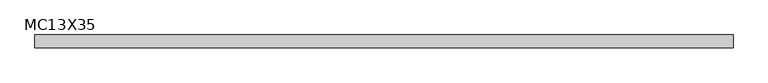
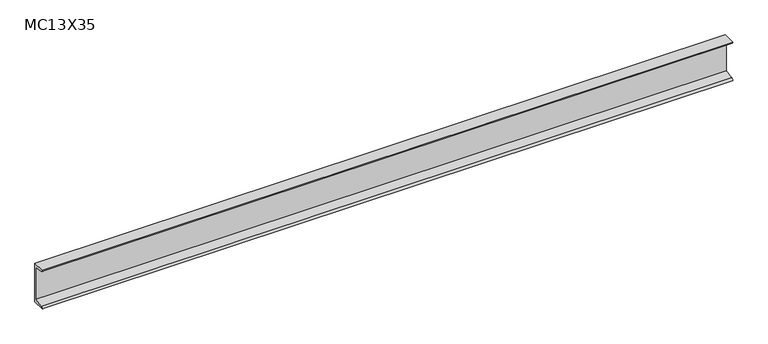
"""IFC4 building model written with IfcOpenShell, lengths in millimetres: beam geometry, MC-Miscellaneous Channel : MC13X35."""

from ifc_helpers import new_model, si_unit, point, frame, frame_2d, origin, place, context, project, spatial, polyline, circle_curve, trimmed, segment, composite_curve, outline, extrude, source, transform, mapped, element, save


def mc13x35_d1883c7b(model_context):
    return source(origin(), model_context, "Body", "SweptSolid", [
        extrude(outline(composite_curve([segment(polyline([(24.892, 165.1), (24.892, -165.1), (-78.486, -165.1)]), True, "CONTINUOUS"), segment(trimmed(circle_curve(frame_2d((-62.992, -165.1)), 15.494), [point((-78.486, -165.1))], [point((-62.992, -149.606))], False, "CARTESIAN"), True, "CONTINUOUS"), segment(polyline([(-62.992, -149.606), (13.5382, -137.4848071), (13.5382, 137.4848071), (-62.992, 149.606)]), True, "CONTINUOUS"), segment(trimmed(circle_curve(frame_2d((-62.992, 165.1)), 15.494), [point((-62.992, 149.606))], [point((-78.486, 165.1))], False, "CARTESIAN"), True, "CONTINUOUS"), segment(polyline([(-78.486, 165.1), (24.892, 165.1)]), True, "CONTINUOUS")], self_intersect=False)), frame((-2806.7, 0.0, 0.0), z_axis=(1.0, 0.0, 0.0), x_axis=(0.0, 1.0, 0.0)), (0.0, 0.0, 1.0), 5613.4),
    ])


if __name__ == "__main__":
    model = new_model("IFC4")
    model_context = context("Model", 3, world=origin())
    ifc_project = project(units=[si_unit("LENGTHUNIT", "METRE", prefix="MILLI")], contexts=[model_context])
    site = spatial("IfcSite", under=ifc_project)
    building = spatial("IfcBuilding", under=site)
    placement = place(None, origin())
    mc13x35_shape = mc13x35_d1883c7b(model_context)
    element("IfcBeam", 1, ObjectType="MC-Miscellaneous Channel : MC13X35", at=placement, inside=building, context=model_context, shape_type="MappedRepresentation", body=[
        mapped(mc13x35_shape, transform((0.0, 0.0, 0.0), x_axis=(1.0, 0.0, 0.0), y_axis=(0.0, 1.0, 0.0), z_axis=(0.0, 0.0, 1.0))),
    ])
    save(model, "model.ifc")

# Revit data of these elements
# Type "MC-Miscellaneous Channel : MC13X35"
#   Assembly Code = "B10"
#   W = 35
#   Length [instance default] = 5' - 0"
#   bf = 0' - 4.07"
#   d = 1' - 1"
#   tf = 0' - 0.61"
#   tw = 0' - 0.447"
#   x = 0' - 0.98"
#   A = 0.0715278 SF
#   Structural Material [instance default] = Steel ASTM A36
# Element 1 (IfcBeam, "MC-Miscellaneous Channel : MC13X35")
#   Structural Material = Steel ASTM A992
#   Materials on its faces: "Steel ASTM A992"
# Materials
#   "Steel ASTM A36": class "Metal", colour RGB 199 199 199, transparency 0, Description = "Structural steel, ASTM A36 Grade B, mill finish", Cost = 0
#   "Steel ASTM A992": class "Metal", colour RGB 199 199 199, transparency 0, Description = "Structural steel 50ksi", Cost = 0
